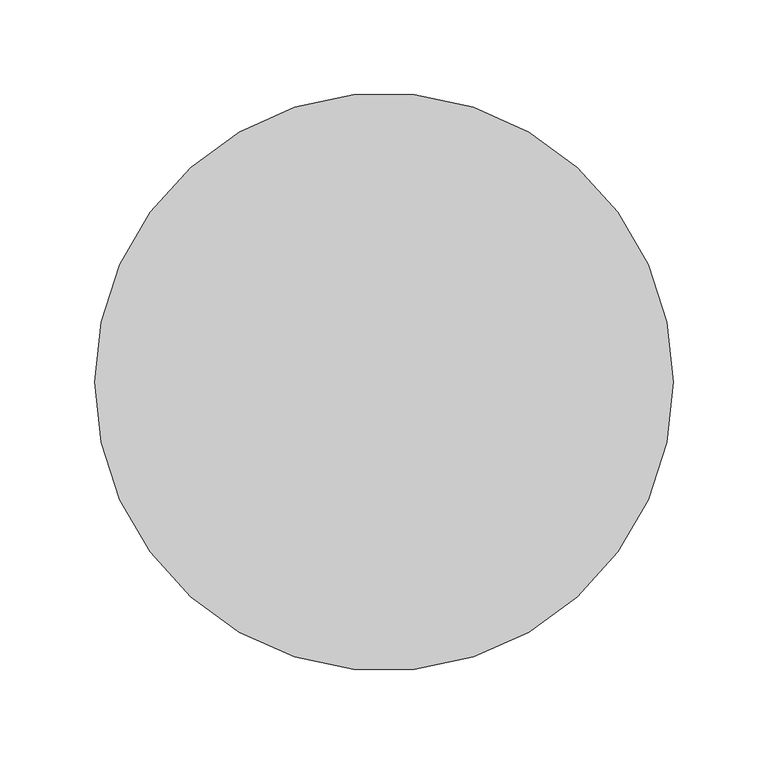
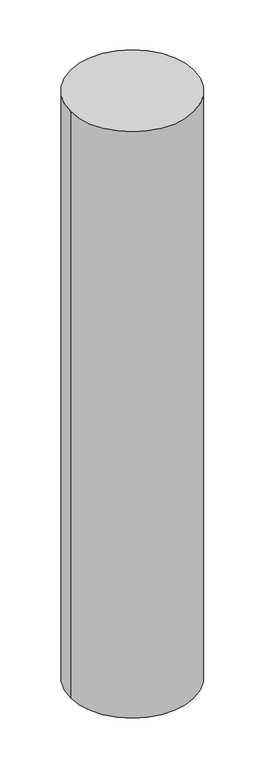
"""IFC4 building model written with IfcOpenShell, lengths in millimetres: proxy geometry."""

from ifc_helpers import new_model, si_unit, point, frame, frame_2d, origin, place, context, project, spatial, circle_curve, trimmed, segment, composite_curve, outline, extrude, source, transform, mapped, element, save


def generic_models_e1c0c775(model_context):
    return source(origin(), model_context, "Body", "SweptSolid", [
        extrude(outline(composite_curve([segment(trimmed(circle_curve(frame_2d((590220.6835267, -534045.8663841)), 152.4), [point((590068.2835267, -534045.8663841))], [point((590373.0835267, -534045.8663841))], False, "CARTESIAN"), True, "CONTINUOUS"), segment(trimmed(circle_curve(frame_2d((590220.6835267, -534045.8663841)), 152.4), [point((590373.0835267, -534045.8663841))], [point((590068.2835267, -534045.8663841))], False, "CARTESIAN"), True, "CONTINUOUS")], self_intersect=False)), frame((0.0, 0.0, -1676.4), z_axis=(0.0, 0.0, 1.0), x_axis=(1.0, 0.0, 0.0)), (0.0, 0.0, 1.0), 1524.0),
    ])


if __name__ == "__main__":
    model = new_model("IFC4")
    model_context = context("Model", 3, world=origin())
    ifc_project = project(units=[si_unit("LENGTHUNIT", "METRE", prefix="MILLI")], contexts=[model_context])
    site = spatial("IfcSite", under=ifc_project)
    building = spatial("IfcBuilding", under=site)
    placement = place(None, origin())
    generic_models_shape = generic_models_e1c0c775(model_context)
    element("IfcBuildingElementProxy", 1, Name="Sonotube Pier 2B : 12\" Sonotube Pier", ObjectType="Sonotube Pier 2B : 12\" Sonotube Pier", at=placement, inside=building, context=model_context, shape_type="MappedRepresentation", body=[
        mapped(generic_models_shape, transform((0.0, 0.0, 0.0), x_axis=(1.0, 0.0, 0.0), y_axis=(0.0, 1.0, 0.0), z_axis=(0.0, 0.0, 1.0))),
    ])
    save(model, "model.ifc")

# Revit data of these elements
# Element 1 (IfcBuildingElementProxy, "Sonotube Pier 2B : 12\" Sonotube Pier")
#   Materials on its faces: "12\" CONC SONOTUBE MIN. 60\" BELOW GRADE"
# Materials
#   "12\" CONC SONOTUBE MIN. 60\" BELOW GRADE": class "Generic", colour RGB 145 145 143, transparency 0, Cost = 0
